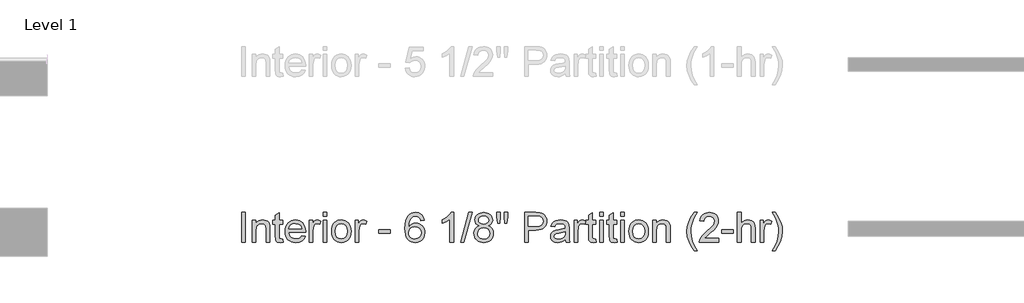
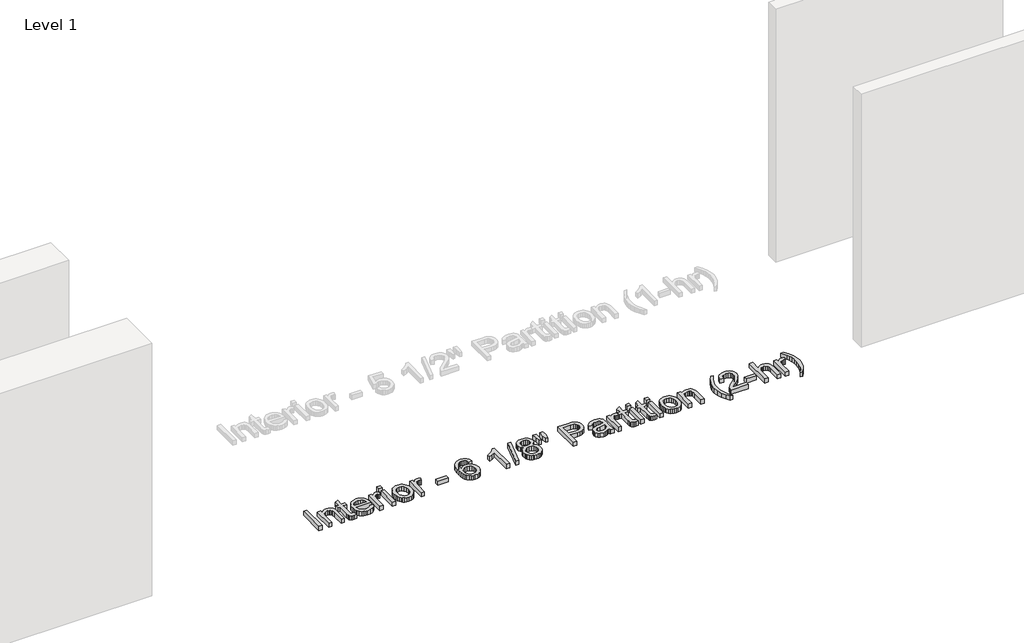
# One storey, part 32 of 42: 1 proxy.
"""IFC4 building model written with IfcOpenShell, lengths in millimetres."""

from ifc_helpers import new_model, si_unit, origin, origin_with_axes, place, context, project, spatial, polyline, outline, extrude, element, save

model = new_model("IFC4")

# Units and contexts
model_context = context("Model", 3, world=origin())
ifc_project = project(units=[si_unit("LENGTHUNIT", "METRE", prefix="MILLI")], contexts=[model_context])

# Site, building, storey
site = spatial("IfcSite", under=ifc_project)
building = spatial("IfcBuilding", under=site)
storey = spatial("IfcBuildingStorey", under=building, Name="Level 1", Elevation=0.0)

# Proxy
placement = place(None, origin())
element("IfcBuildingElementProxy", 1, Name="8\" Arial", ObjectType="8\" Arial", at=placement, inside=storey, context=model_context, shape_type="SweptSolid", body=[
    extrude(outline(polyline([(5266.6577476, 8426.7514962), (5266.6577476, 8731.3185903), (5304.7286344, 8731.3185903), (5304.7286344, 8426.7514962), (5266.6577476, 8426.7514962)])), origin_with_axes(), (0.0, 0.0, 1.0), 50.8),
    extrude(outline(polyline([(5376.111547, 8426.7514962), (5376.111547, 8650.4179559), (5414.1824338, 8650.4179559), (5414.1824338, 8619.1879316), (5427.4087209, 8634.9330688), (5443.2932779, 8646.1795955), (5461.8361048, 8652.9275114), (5483.0372016, 8655.1768167), (5501.8031002, 8653.36436), (5518.9889082, 8647.9269897), (5533.3212586, 8639.5432153), (5543.5267844, 8628.8915463), (5554.9406147, 8600.8960602), (5556.9482591, 8564.0892459), (5556.9482591, 8426.7514962), (5518.8773724, 8426.7514962), (5518.8773724, 8558.958599), (5514.4902975, 8592.6424109), (5508.420891, 8602.6713384), (5498.9868212, 8610.4509605), (5486.8944814, 8615.4421876), (5472.8502651, 8617.10593), (5450.5523996, 8613.3694806), (5431.5448402, 8602.1601326), (5423.9487874, 8593.0095496), (5418.5230354, 8580.5035979), (5414.1824338, 8545.4255885), (5414.1824338, 8426.7514962), (5376.111547, 8426.7514962)])), origin_with_axes(), (0.0, 0.0, 1.0), 50.8),
    extrude(outline(polyline([(5690.1963628, 8458.5020209), (5694.9552236, 8425.6361382), (5666.4764158, 8421.9926353), (5648.2031337, 8423.5727259), (5634.5771767, 8428.3129974), (5624.9479192, 8435.6185924), (5618.6647357, 8444.8946532), (5615.2071259, 8460.8256834), (5614.0545893, 8488.0961868), (5614.0545893, 8612.3470691), (5585.5014242, 8612.3470691), (5585.5014242, 8650.4179559), (5614.0545893, 8650.4179559), (5614.0545893, 8704.7730696), (5652.125476, 8727.154587), (5652.125476, 8650.4179559), (5690.1963628, 8650.4179559), (5690.1963628, 8612.3470691), (5652.125476, 8612.3470691), (5652.125476, 8489.2115448), (5654.1331204, 8469.5812438), (5660.6393755, 8462.6288455), (5673.614707, 8460.0635221), (5690.1963628, 8458.5020209)])), origin_with_axes(), (0.0, 0.0, 1.0), 50.8),
    extrude(outline(polyline([(5884.8635142, 8493.375548), (5922.190829, 8488.6166872), (5908.7414703, 8460.491076), (5887.2801232, 8439.4665775), (5858.2901096, 8426.3611209), (5822.2547512, 8421.9926353), (5798.632398, 8423.8771256), (5777.5846629, 8429.5305966), (5759.1115459, 8438.9530481), (5743.2130469, 8452.1444802), (5730.4282557, 8468.7377543), (5721.296262, 8488.3657316), (5715.8170658, 8511.0284122), (5713.990667, 8536.725796), (5715.8356551, 8563.2945533), (5721.3706192, 8586.7124242), (5730.5955594, 8606.9794087), (5743.5104757, 8624.0955068), (5759.3671487, 8637.6935799), (5777.4173592, 8647.4064893), (5797.6611071, 8653.2342349), (5820.0983924, 8655.1768167), (5841.8130187, 8653.2388822), (5861.4502907, 8647.4250786), (5879.0102083, 8637.7354058), (5894.4927717, 8624.169864), (5907.1311722, 8607.0909445), (5916.1586011, 8586.8611386), (5921.5750584, 8563.4804463), (5923.3805442, 8536.9488676), (5923.1574726, 8526.6875739), (5752.0615538, 8526.6875739), (5758.6514607, 8498.1901768), (5773.9597494, 8477.2400355), (5796.0531326, 8464.3576504), (5822.9983232, 8460.0635221), (5843.2606604, 8462.0525772), (5860.325638, 8468.0197426), (5874.1932559, 8478.3368042), (5884.8635142, 8493.375548)]), holes=[polyline([(5752.0615538, 8564.7584607), (5885.3096574, 8564.7584607), (5880.1604213, 8584.8720835), (5870.0664313, 8599.2602018), (5847.8708069, 8612.6444979), (5819.949678, 8617.10593), (5794.2871491, 8613.546079), (5773.067463, 8602.866526), (5758.3168533, 8586.2198077), (5752.0615538, 8564.7584607)])]), origin_with_axes(), (0.0, 0.0, 1.0), 50.8),
    extrude(outline(polyline([(5961.4514309, 8426.7514962), (5961.4514309, 8650.4179559), (5994.7634569, 8650.4179559), (5994.7634569, 8617.3290016), (6007.0695736, 8636.5131594), (6018.4090467, 8647.8154539), (6029.7856984, 8653.336476), (6042.2033509, 8655.1768167), (6061.1644371, 8652.2397073), (6080.4229521, 8643.428379), (6067.7078707, 8609.2984239), (6054.3235746, 8615.1540535), (6040.9392785, 8617.10593), (6029.5719214, 8615.2284107), (6019.4128689, 8609.5958527), (6011.2056929, 8600.63581), (6005.6939654, 8588.7758365), (6001.0652296, 8567.5096771), (5999.5223177, 8544.3102305), (5999.5223177, 8426.7514962), (5961.4514309, 8426.7514962)])), origin_with_axes(), (0.0, 0.0, 1.0), 50.8),
    extrude(outline(polyline([(6104.2172563, 8693.2477035), (6104.2172563, 8731.3185903), (6142.288143, 8731.3185903), (6142.288143, 8693.2477035), (6104.2172563, 8693.2477035)])), origin_with_axes(), (0.0, 0.0, 1.0), 50.8),
    extrude(outline(polyline([(6104.2172563, 8426.7514962), (6104.2172563, 8650.4179559), (6142.288143, 8650.4179559), (6142.288143, 8426.7514962), (6104.2172563, 8426.7514962)])), origin_with_axes(), (0.0, 0.0, 1.0), 50.8),
    extrude(outline(polyline([(6189.8767515, 8538.584726), (6191.9355165, 8567.551503), (6198.1118115, 8592.5122858), (6208.4056364, 8613.4670745), (6222.8169914, 8630.4158689), (6237.3259402, 8641.2487836), (6253.3406223, 8648.9865798), (6270.8610377, 8653.6292575), (6289.8871864, 8655.1768167), (6310.890772, 8653.2923264), (6329.8820658, 8647.6388555), (6346.8610678, 8638.216404), (6361.8277781, 8625.0249719), (6374.043272, 8608.5107023), (6382.7686248, 8589.1197386), (6388.0038364, 8566.8520806), (6389.748907, 8541.7077285), (6386.6630831, 8503.2464664), (6377.4056117, 8473.9683186), (6362.2460374, 8452.0422391), (6341.4539051, 8435.6371817), (6316.7580198, 8425.4037719), (6289.8871864, 8421.9926353), (6268.5768774, 8423.8701547), (6249.4089853, 8429.5027126), (6232.38351, 8438.8903092), (6217.5004516, 8452.0329444), (6205.4150828, 8468.7075467), (6196.7826765, 8488.6910444), (6191.6032327, 8511.9834375), (6189.8767515, 8538.584726)]), holes=[polyline([(6227.9476383, 8538.6590832), (6232.3533024, 8504.2038154), (6245.5702948, 8479.6566445), (6265.460846, 8464.9618027), (6289.8871864, 8460.0635221), (6314.2019911, 8464.9896866), (6334.0553637, 8479.7681803), (6347.2723561, 8504.6406639), (6351.6780202, 8539.8487985), (6347.2444721, 8573.3002441), (6333.9438279, 8597.5128076), (6314.0625713, 8612.2076494), (6289.8871864, 8617.10593), (6265.460846, 8612.2262387), (6245.5702948, 8597.5871648), (6232.3533024, 8573.0957618), (6227.9476383, 8538.6590832)])]), origin_with_axes(), (0.0, 0.0, 1.0), 50.8),
    extrude(outline(polyline([(6432.5786546, 8426.7514962), (6432.5786546, 8650.4179559), (6465.8906805, 8650.4179559), (6465.8906805, 8617.3290016), (6478.1967972, 8636.5131594), (6489.5362703, 8647.8154539), (6500.912922, 8653.336476), (6513.3305745, 8655.1768167), (6532.2916607, 8652.2397073), (6551.5501757, 8643.428379), (6538.8350944, 8609.2984239), (6525.4507983, 8615.1540535), (6512.0665021, 8617.10593), (6500.6991451, 8615.2284107), (6490.5400925, 8609.5958527), (6482.3329165, 8600.63581), (6476.821189, 8588.7758365), (6472.1924533, 8567.5096771), (6470.6495413, 8544.3102305), (6470.6495413, 8426.7514962), (6432.5786546, 8426.7514962)])), origin_with_axes(), (0.0, 0.0, 1.0), 50.8),
    extrude(outline(polyline([(6675.2805577, 8517.1698522), (6675.2805577, 8555.240739), (6794.2520788, 8555.240739), (6794.2520788, 8517.1698522), (6675.2805577, 8517.1698522)])), origin_with_axes(), (0.0, 0.0, 1.0), 50.8),
    extrude(outline(polyline([(7141.6489205, 8650.4179559), (7103.5780337, 8645.659095), (7097.4435646, 8664.5272347), (7089.1527368, 8677.4096197), (7071.8832769, 8689.2881826), (7051.0074928, 8693.2477035), (7033.310479, 8690.9426303), (7016.6544661, 8684.0274106), (7002.3499996, 8669.4626939), (6990.6666244, 8649.4141337), (6982.7754665, 8621.0561563), (6979.8476517, 8581.563188), (6995.1187618, 8599.3810323), (7013.4199278, 8611.9381045), (7033.7287383, 8619.3831193), (7055.0227816, 8621.8647908), (7073.314653, 8620.1685172), (7090.1937376, 8615.0796963), (7105.6600353, 8606.5983281), (7119.7135463, 8594.7244126), (7131.3922741, 8580.1643432), (7139.7342225, 8563.6245134), (7144.7393916, 8545.1049231), (7146.4077813, 8524.6055723), (7143.2661896, 8497.3443636), (7133.8414144, 8472.07221), (7118.9142063, 8450.6387469), (7099.2653161, 8434.8936097), (7075.7870299, 8425.2178789), (7049.3716344, 8421.9926353), (7026.6764225, 8424.1304049), (7006.1793954, 8430.5437134), (6987.8805531, 8441.232561), (6971.7798955, 8456.1969477), (6958.6535259, 8476.0689096), (6949.2775476, 8501.4804829), (6943.6519606, 8532.4316677), (6941.776765, 8568.9224639), (6943.8587666, 8609.8328663), (6950.1047715, 8644.7482193), (6960.5147796, 8673.6685231), (6975.0887909, 8696.5937775), (6990.8850487, 8711.7858831), (7009.2001567, 8722.6373871), (7030.0341149, 8729.1482895), (7053.3869232, 8731.3185903), (7086.7918956, 8725.9462825), (7113.5418986, 8709.8293593), (7132.2799132, 8684.2318929), (7141.6489205, 8650.4179559)]), holes=[polyline([(6979.8476517, 8525.2004299), (6982.0504838, 8508.33064), (6988.65898, 8492.2230114), (6998.9202737, 8478.3739828), (7012.0814982, 8468.2799928), (7027.9660552, 8462.1176398), (7046.3973464, 8460.0635221), (7071.5207855, 8464.3204718), (7091.271917, 8477.0913211), (7104.0706502, 8497.1677652), (7108.3368945, 8523.3414999), (7104.1264181, 8548.4649391), (7091.4949886, 8567.6212129), (7071.4092497, 8579.7507313), (7044.8358451, 8583.7939041), (7019.7495846, 8579.7507313), (6998.7715593, 8567.6212129), (6984.5786286, 8548.9296716), (6979.8476517, 8525.2004299)])]), origin_with_axes(), (0.0, 0.0, 1.0), 50.8),
    extrude(outline(polyline([(7441.4571537, 8426.7514962), (7403.3862669, 8426.7514962), (7403.3862669, 8664.0996808), (7367.3230246, 8638.409268), (7327.2444934, 8619.1879316), (7327.2444934, 8655.1768167), (7357.1453827, 8671.4424544), (7383.0495725, 8690.7939159), (7403.4699188, 8711.3722712), (7416.9192774, 8731.3185903), (7441.4571537, 8731.3185903), (7441.4571537, 8426.7514962)])), origin_with_axes(), (0.0, 0.0, 1.0), 50.8),
    extrude(outline(polyline([(7512.8400664, 8426.7514962), (7598.4995616, 8731.3185903), (7632.8525883, 8731.3185903), (7547.1930931, 8426.7514962), (7512.8400664, 8426.7514962)])), origin_with_axes(), (0.0, 0.0, 1.0), 50.8),
    extrude(outline(polyline([(7706.3175026, 8594.501341), (7685.9343349, 8604.5395631), (7671.6298684, 8618.1469308), (7663.1810315, 8635.0446046), (7660.3647525, 8654.9537451), (7661.8983698, 8670.4804581), (7666.4992216, 8684.7152147), (7674.1673079, 8697.658015), (7684.9026288, 8709.3088588), (7698.1893311, 8718.9381163), (7713.5115617, 8725.8161574), (7750.2626082, 8731.3185903), (7787.2367262, 8725.6860323), (7802.7262606, 8718.6453349), (7816.2174452, 8708.7883584), (7827.1479537, 8696.9097956), (7834.9554598, 8683.804339), (7839.6399634, 8669.4719886), (7841.2014646, 8653.9127443), (7838.4223643, 8634.6449347), (7830.0850631, 8618.035395), (7816.0966148, 8604.5116791), (7796.3640726, 8594.501341), (7819.7958855, 8582.4275905), (7836.8515684, 8564.6469249), (7847.2522819, 8542.0144519), (7850.7191863, 8515.3852794), (7848.9996761, 8496.3963093), (7843.8411453, 8478.9874297), (7835.2435939, 8463.1586406), (7823.2070221, 8448.909942), (7808.3634659, 8437.1336203), (7791.3449616, 8428.721962), (7772.1515091, 8423.674967), (7750.7831086, 8421.9926353), (7729.414708, 8423.681938), (7710.2212556, 8428.749846), (7693.2027513, 8437.1963592), (7678.3591951, 8449.0214778), (7666.3226232, 8463.3700939), (7657.7250719, 8479.3870996), (7652.5665411, 8497.0724951), (7650.8470309, 8516.4262802), (7654.4533551, 8544.0871589), (7665.2723278, 8566.8404623), (7682.74627, 8583.9054399), (7706.3175026, 8594.501341)]), holes=[polyline([(7688.9179176, 8517.7647098), (7690.5073028, 8503.1999932), (7695.2754583, 8489.100009), (7704.0774919, 8476.8031869), (7717.7685115, 8467.6479566), (7734.1642742, 8461.9596307), (7751.0805374, 8460.0635221), (7776.9940218, 8464.050927), (7796.4384298, 8476.0131417), (7808.5958321, 8494.1284147), (7812.6482996, 8516.5749946), (7808.465707, 8539.4026552), (7795.9179294, 8557.9175982), (7776.0273782, 8570.1865363), (7749.816465, 8574.2761824), (7724.2654719, 8570.2423042), (7705.0162516, 8558.1406698), (7692.9425011, 8539.9789236), (7688.9179176, 8517.7647098)]), polyline([(7698.4356393, 8653.8383871), (7701.8095973, 8637.2195528), (7711.9314712, 8623.9467924), (7728.5038323, 8615.247), (7751.2292518, 8612.3470691), (7773.4248762, 8615.2284107), (7789.7462818, 8623.8724352), (7799.7845039, 8636.6990524), (7803.1305779, 8652.1281715), (7799.6729681, 8668.1428536), (7789.3001386, 8681.38773), (7772.7556614, 8690.2827101), (7750.7831086, 8693.2477035), (7728.671136, 8690.3477727), (7712.1545428, 8681.6479802), (7701.8653652, 8668.8957203), (7698.4356393, 8653.8383871)])]), origin_with_axes(), (0.0, 0.0, 1.0), 50.8),
    extrude(outline(polyline([(7893.3258623, 8621.8647908), (7884.0312122, 8680.6813366), (7884.0312122, 8731.3185903), (7922.102099, 8731.3185903), (7922.102099, 8680.6813366), (7913.7740925, 8621.8647908), (7893.3258623, 8621.8647908)])), origin_with_axes(), (0.0, 0.0, 1.0), 50.8),
    extrude(outline(polyline([(7969.2445643, 8621.8647908), (7960.1729858, 8680.6813366), (7960.1729858, 8731.3185903), (7998.2438725, 8731.3185903), (7998.2438725, 8680.6813366), (7989.3210084, 8621.8647908), (7969.2445643, 8621.8647908)])), origin_with_axes(), (0.0, 0.0, 1.0), 50.8),
    extrude(outline(polyline([(8169.5628629, 8426.7514962), (8169.5628629, 8731.3185903), (8282.4370936, 8731.3185903), (8327.9437004, 8728.4186594), (8348.2339216, 8722.9998784), (8364.9364078, 8714.1792555), (8378.3857665, 8701.5571207), (8388.916605, 8684.733804), (8395.7202889, 8664.8897261), (8397.9881835, 8643.2053074), (8396.4568899, 8624.5091188), (8391.8630091, 8607.3093688), (8384.2065411, 8591.6060575), (8373.4874859, 8577.3991848), (8358.7717311, 8565.6228631), (8339.1251645, 8557.2112048), (8314.547786, 8552.1642098), (8285.0395956, 8550.4818782), (8207.6337497, 8550.4818782), (8207.6337497, 8426.7514962), (8169.5628629, 8426.7514962)]), holes=[polyline([(8207.6337497, 8588.5527649), (8287.2703116, 8588.5527649), (8321.0284808, 8592.0475533), (8343.335641, 8602.5319186), (8355.7718828, 8619.3552353), (8359.9172967, 8641.8668778), (8357.4728038, 8658.969034), (8350.1393248, 8673.3943309), (8338.8277357, 8684.2504822), (8324.448912, 8690.6452015), (8286.3780252, 8693.2477035), (8207.6337497, 8693.2477035), (8207.6337497, 8588.5527649)])]), origin_with_axes(), (0.0, 0.0, 1.0), 50.8),
    extrude(outline(polyline([(8588.3426173, 8455.3046613), (8570.1529871, 8439.7082384), (8551.4242671, 8429.5027126), (8531.7289036, 8423.8701547), (8510.6393426, 8421.9926353), (8478.8237553, 8426.5098353), (8455.3547638, 8440.0614351), (8440.8829936, 8460.6397904), (8436.0590702, 8486.2372567), (8437.8808217, 8502.0195726), (8443.3460759, 8516.351923), (8451.7763235, 8528.6208611), (8462.4930551, 8538.21294), (8489.1501115, 8550.7049498), (8522.0903515, 8556.4304542), (8561.016346, 8562.4533875), (8588.1195457, 8569.5173215), (8588.3426173, 8577.9940424), (8585.721526, 8594.9846628), (8577.858252, 8606.1010643), (8560.272774, 8614.3547136), (8535.7720764, 8617.10593), (8513.0931302, 8615.2748839), (8497.2550464, 8609.7817457), (8486.454663, 8599.6226932), (8478.8888179, 8583.7939041), (8440.8179311, 8588.5527649), (8447.4264273, 8609.3727811), (8457.288051, 8625.7313653), (8471.3229727, 8638.2419643), (8490.4513626, 8647.5180251), (8513.8459968, 8653.2621188), (8540.6796516, 8655.1768167), (8566.4165377, 8653.4851904), (8586.8182947, 8648.4103115), (8602.2009406, 8640.7794038), (8612.8804935, 8631.4196911), (8619.9630169, 8619.8478518), (8624.554574, 8605.5805639), (8626.413504, 8572.268538), (8626.413504, 8524.9030011), (8628.3467913, 8458.7622711), (8635.9312257, 8426.7514962), (8597.860339, 8426.7514962), (8591.7630485, 8439.9870779), (8588.3426173, 8455.3046613)]), holes=[polyline([(8588.3426173, 8531.4464348), (8526.9235695, 8519.7723543), (8494.1692226, 8513.6007066), (8479.3349611, 8503.5624845), (8474.129957, 8488.914116), (8476.9648253, 8477.5932322), (8485.4694301, 8468.3171714), (8499.4578785, 8462.1269344), (8518.7442774, 8460.0635221), (8539.1925076, 8462.3407114), (8557.2613074, 8469.1722792), (8571.9096759, 8479.2383852), (8582.0966124, 8491.2191892), (8586.6138124, 8503.5624845), (8588.1195457, 8520.6646407), (8588.3426173, 8531.4464348)])]), origin_with_axes(), (0.0, 0.0, 1.0), 50.8),
    extrude(outline(polyline([(8678.7609733, 8426.7514962), (8678.7609733, 8650.4179559), (8712.0729992, 8650.4179559), (8712.0729992, 8617.3290016), (8724.379116, 8636.5131594), (8735.7185891, 8647.8154539), (8747.0952408, 8653.336476), (8759.5128933, 8655.1768167), (8778.4739795, 8652.2397073), (8797.7324945, 8643.428379), (8785.0174131, 8609.2984239), (8771.633117, 8615.1540535), (8758.2488209, 8617.10593), (8746.8814638, 8615.2284107), (8736.7224113, 8609.5958527), (8728.5152353, 8600.63581), (8723.0035078, 8588.7758365), (8718.374772, 8567.5096771), (8716.8318601, 8544.3102305), (8716.8318601, 8426.7514962), (8678.7609733, 8426.7514962)])), origin_with_axes(), (0.0, 0.0, 1.0), 50.8),
    extrude(outline(polyline([(8902.427433, 8458.5020209), (8907.1862939, 8425.6361382), (8878.707486, 8421.9926353), (8860.4342039, 8423.5727259), (8846.8082469, 8428.3129974), (8837.1789894, 8435.6185924), (8830.895806, 8444.8946532), (8827.4381961, 8460.8256834), (8826.2856595, 8488.0961868), (8826.2856595, 8612.3470691), (8797.7324945, 8612.3470691), (8797.7324945, 8650.4179559), (8826.2856595, 8650.4179559), (8826.2856595, 8704.7730696), (8864.3565463, 8727.154587), (8864.3565463, 8650.4179559), (8902.427433, 8650.4179559), (8902.427433, 8612.3470691), (8864.3565463, 8612.3470691), (8864.3565463, 8489.2115448), (8866.3641907, 8469.5812438), (8872.8704458, 8462.6288455), (8885.8457773, 8460.0635221), (8902.427433, 8458.5020209)])), origin_with_axes(), (0.0, 0.0, 1.0), 50.8),
    extrude(outline(polyline([(8940.4983198, 8693.2477035), (8940.4983198, 8731.3185903), (8978.5692066, 8731.3185903), (8978.5692066, 8693.2477035), (8940.4983198, 8693.2477035)])), origin_with_axes(), (0.0, 0.0, 1.0), 50.8),
    extrude(outline(polyline([(8940.4983198, 8426.7514962), (8940.4983198, 8650.4179559), (8978.5692066, 8650.4179559), (8978.5692066, 8426.7514962), (8940.4983198, 8426.7514962)])), origin_with_axes(), (0.0, 0.0, 1.0), 50.8),
    extrude(outline(polyline([(9116.5761711, 8458.5020209), (9121.3350319, 8425.6361382), (9092.856224, 8421.9926353), (9074.582942, 8423.5727259), (9060.9569849, 8428.3129974), (9051.3277274, 8435.6185924), (9045.044544, 8444.8946532), (9041.5869342, 8460.8256834), (9040.4343975, 8488.0961868), (9040.4343975, 8612.3470691), (9011.8812325, 8612.3470691), (9011.8812325, 8650.4179559), (9040.4343975, 8650.4179559), (9040.4343975, 8704.7730696), (9078.5052843, 8727.154587), (9078.5052843, 8650.4179559), (9116.5761711, 8650.4179559), (9116.5761711, 8612.3470691), (9078.5052843, 8612.3470691), (9078.5052843, 8489.2115448), (9080.5129287, 8469.5812438), (9087.0191838, 8462.6288455), (9099.9945153, 8460.0635221), (9116.5761711, 8458.5020209)])), origin_with_axes(), (0.0, 0.0, 1.0), 50.8),
    extrude(outline(polyline([(9154.6470578, 8426.7514962), (9154.6470578, 8650.4179559), (9192.7179446, 8650.4179559), (9192.7179446, 8426.7514962), (9154.6470578, 8426.7514962)])), origin_with_axes(), (0.0, 0.0, 1.0), 50.8),
    extrude(outline(polyline([(9154.6470578, 8693.2477035), (9154.6470578, 8731.3185903), (9192.7179446, 8731.3185903), (9192.7179446, 8693.2477035), (9154.6470578, 8693.2477035)])), origin_with_axes(), (0.0, 0.0, 1.0), 50.8),
    extrude(outline(polyline([(9240.306553, 8538.584726), (9242.365318, 8567.551503), (9248.541613, 8592.5122858), (9258.835438, 8613.4670745), (9273.2467929, 8630.4158689), (9287.7557417, 8641.2487836), (9303.7704238, 8648.9865798), (9321.2908392, 8653.6292575), (9340.316988, 8655.1768167), (9361.3205735, 8653.2923264), (9380.3118673, 8647.6388555), (9397.2908693, 8638.216404), (9412.2575796, 8625.0249719), (9424.4730735, 8608.5107023), (9433.1984263, 8589.1197386), (9438.433638, 8566.8520806), (9440.1787085, 8541.7077285), (9437.0928847, 8503.2464664), (9427.8354132, 8473.9683186), (9412.6758389, 8452.0422391), (9391.8837066, 8435.6371817), (9367.1878214, 8425.4037719), (9340.316988, 8421.9926353), (9319.006679, 8423.8701547), (9299.8387868, 8429.5027126), (9282.8133115, 8438.8903092), (9267.9302531, 8452.0329444), (9255.8448843, 8468.7075467), (9247.212478, 8488.6910444), (9242.0330343, 8511.9834375), (9240.306553, 8538.584726)]), holes=[polyline([(9278.3774398, 8538.6590832), (9282.7831039, 8504.2038154), (9296.0000963, 8479.6566445), (9315.8906475, 8464.9618027), (9340.316988, 8460.0635221), (9364.6317926, 8464.9896866), (9384.4851652, 8479.7681803), (9397.7021576, 8504.6406639), (9402.1078217, 8539.8487985), (9397.6742737, 8573.3002441), (9384.3736294, 8597.5128076), (9364.4923728, 8612.2076494), (9340.316988, 8617.10593), (9315.8906475, 8612.2262387), (9296.0000963, 8597.5871648), (9282.7831039, 8573.0957618), (9278.3774398, 8538.6590832)])]), origin_with_axes(), (0.0, 0.0, 1.0), 50.8),
    extrude(outline(polyline([(9483.0084561, 8426.7514962), (9483.0084561, 8650.4179559), (9521.0793429, 8650.4179559), (9521.0793429, 8619.1879316), (9534.3056299, 8634.9330688), (9550.1901869, 8646.1795955), (9568.7330139, 8652.9275114), (9589.9341107, 8655.1768167), (9608.7000092, 8653.36436), (9625.8858173, 8647.9269897), (9640.2181677, 8639.5432153), (9650.4236935, 8628.8915463), (9661.8375238, 8600.8960602), (9663.8451682, 8564.0892459), (9663.8451682, 8426.7514962), (9625.7742815, 8426.7514962), (9625.7742815, 8558.958599), (9621.3872066, 8592.6424109), (9615.3178001, 8602.6713384), (9605.8837303, 8610.4509605), (9593.7913905, 8615.4421876), (9579.7471742, 8617.10593), (9557.4493087, 8613.3694806), (9538.4417492, 8602.1601326), (9530.8456964, 8593.0095496), (9525.4199445, 8580.5035979), (9521.0793429, 8545.4255885), (9521.0793429, 8426.7514962), (9483.0084561, 8426.7514962)])), origin_with_axes(), (0.0, 0.0, 1.0), 50.8),
    extrude(outline(polyline([(9911.3059321, 8341.092001), (9881.8047128, 8382.4903725), (9857.2482472, 8430.394999), (9840.6851808, 8482.4822181), (9835.1641586, 8536.4283672), (9839.2909833, 8583.7381362), (9851.6714572, 8629.0030821), (9876.246512, 8680.272372), (9911.3059321, 8731.3185903), (9939.8590972, 8731.3185903), (9904.2419981, 8671.0149005), (9882.8271243, 8612.5701407), (9875.6330651, 8574.4806647), (9873.2350454, 8536.2052956), (9877.3990486, 8487.399088), (9889.8910583, 8438.6114697), (9910.7110745, 8389.8424407), (9939.8590972, 8341.092001), (9911.3059321, 8341.092001)])), origin_with_axes(), (0.0, 0.0, 1.0), 50.8),
    extrude(outline(polyline([(10163.5255569, 8464.8223829), (10163.5255569, 8426.7514962), (9963.6534014, 8426.7514962), (9967.7430475, 8452.999588), (9977.1306441, 8473.5128808), (9990.8681369, 8493.4127266), (10010.7400988, 8514.2420375), (10038.5311025, 8537.5437252), (10079.6134559, 8574.0345215), (10104.262868, 8600.9704174), (10116.587574, 8622.8314344), (10120.6958093, 8644.0975938), (10116.8199402, 8663.1609212), (10105.192333, 8679.0082996), (10087.3187208, 8689.6878525), (10064.7048372, 8693.2477035), (10040.9570062, 8689.7715044), (10022.5071258, 8679.342907), (10010.600679, 8662.7798405), (10006.483149, 8640.9002342), (9968.4122623, 8645.659095), (9971.6863028, 8665.3126327), (9977.6418498, 8682.4844987), (9986.2789034, 8697.1746932), (9997.5974636, 8709.383216), (10011.33728, 8718.9799423), (10027.2381027, 8725.8347467), (10065.5227664, 8731.3185903), (10085.926847, 8729.7942676), (10104.0862696, 8725.2212998), (10120.0010342, 8717.5996867), (10133.6711408, 8706.9294284), (10144.6504463, 8694.0005702), (10152.4928073, 8679.6031572), (10157.1982239, 8663.7371895), (10158.7666961, 8646.4026671), (10157.0750698, 8628.1944475), (10152.0001908, 8610.3022461), (10142.9936749, 8592.1033212), (10129.5071376, 8572.9749314), (10108.0086119, 8550.1379761), (10074.9661309, 8520.8133551), (10031.1697397, 8484.1924337), (10013.9932263, 8464.8223829), (10163.5255569, 8464.8223829)])), origin_with_axes(), (0.0, 0.0, 1.0), 50.8),
    extrude(outline(polyline([(10192.078722, 8517.1698522), (10192.078722, 8555.240739), (10311.0502431, 8555.240739), (10311.0502431, 8517.1698522), (10192.078722, 8517.1698522)])), origin_with_axes(), (0.0, 0.0, 1.0), 50.8),
    extrude(outline(polyline([(10353.8799907, 8426.7514962), (10353.8799907, 8731.3185903), (10391.9508775, 8731.3185903), (10391.9508775, 8619.336646), (10405.9346785, 8635.0167207), (10421.6379898, 8646.2167741), (10439.0608114, 8652.9368061), (10458.2031433, 8655.1768167), (10481.1981076, 8652.7323238), (10500.9585337, 8645.3988448), (10516.5177779, 8633.7526483), (10526.9091967, 8618.3700024), (10532.7648263, 8597.2339681), (10534.7167028, 8568.3276063), (10534.7167028, 8426.7514962), (10496.6458161, 8426.7514962), (10496.6458161, 8564.3866747), (10493.6157601, 8588.2181575), (10484.5255923, 8604.5395631), (10469.8772238, 8613.9643382), (10450.1725656, 8617.10593), (10434.0835263, 8614.9867498), (10418.9797199, 8608.6292091), (10406.4691209, 8598.6467549), (10398.1597037, 8585.6528341), (10393.503084, 8568.3833742), (10391.9508775, 8545.5743029), (10391.9508775, 8426.7514962), (10353.8799907, 8426.7514962)])), origin_with_axes(), (0.0, 0.0, 1.0), 50.8),
    extrude(outline(polyline([(10587.0641721, 8426.7514962), (10587.0641721, 8650.4179559), (10620.376198, 8650.4179559), (10620.376198, 8617.3290016), (10632.6823147, 8636.5131594), (10644.0217878, 8647.8154539), (10655.3984395, 8653.336476), (10667.8160921, 8655.1768167), (10686.7771782, 8652.2397073), (10706.0356932, 8643.428379), (10693.3206119, 8609.2984239), (10679.9363158, 8615.1540535), (10666.5520197, 8617.10593), (10655.1846626, 8615.2284107), (10645.0256101, 8609.5958527), (10636.818434, 8600.63581), (10631.3067065, 8588.7758365), (10626.6779708, 8567.5096771), (10625.1350589, 8544.3102305), (10625.1350589, 8426.7514962), (10587.0641721, 8426.7514962)])), origin_with_axes(), (0.0, 0.0, 1.0), 50.8),
    extrude(outline(polyline([(10739.3477191, 8341.092001), (10710.7945541, 8341.092001), (10739.9425767, 8389.8424407), (10760.7625929, 8438.6114697), (10773.2546027, 8487.399088), (10777.4186059, 8536.2052956), (10775.0205862, 8574.2018252), (10767.826527, 8611.9009259), (10758.7363592, 8641.7739313), (10746.6347248, 8670.4200429), (10710.7945541, 8731.3185903), (10739.3477191, 8731.3185903), (10774.4071393, 8680.272372), (10798.9821941, 8629.0030821), (10811.362668, 8583.7381362), (10815.4894927, 8536.4283672), (10809.9405866, 8482.4822181), (10793.2938682, 8430.394999), (10768.7095188, 8382.4903725), (10739.3477191, 8341.092001)])), origin_with_axes(), (0.0, 0.0, 1.0), 50.8),
])

save(model, "model.ifc")

# Revit data of these elements
# Element 1 (IfcBuildingElementProxy, "8\" Arial")
#   Phase Created = New Construction
